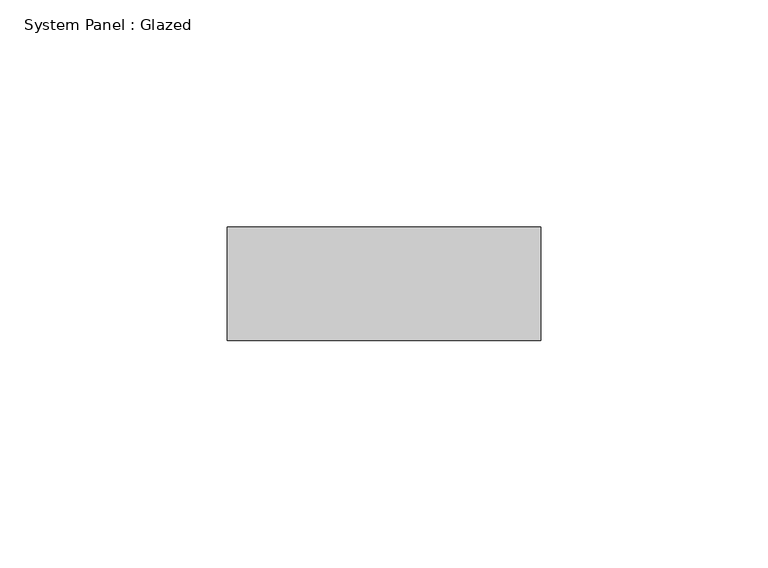
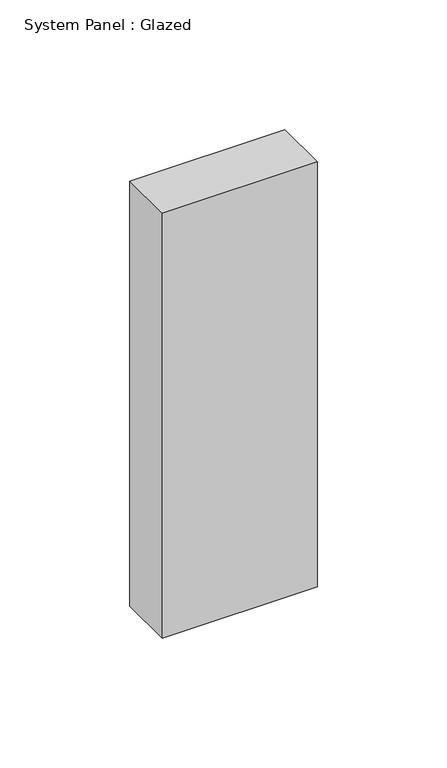
"""IFC4 building model written with IfcOpenShell, lengths in millimetres: plate geometry, System Panel : Glazed."""

import ifcopenshell
import ifcopenshell.guid

model = None  # the IFC model being written
_history = None  # IfcOwnerHistory: only IFC2X3 demands one
_inside = {}  # id of a spatial element -> (the spatial element, [elements in it])
_under = {}  # id of a project, library or spatial element -> (it, [spatial elements below it])
_declared = {}  # id of a project -> (the project, [libraries it declares])
_typed = {}  # id of a type object -> (the type object, [elements of that type])
_made_of = {}  # id of a material, layer set ... -> (it, [elements and type objects made of it])


def new_model(schema):
    """Start an empty IFC model of exactly this schema.

    Asked for "IFC4X3", IfcOpenShell would pick the latest addendum, in which some entities
    have other attributes; the version numbers below select the first issue.
    IFC2X3 requires an IfcOwnerHistory on every rooted entity: one is made here for all.
    """
    global model, _history
    if schema == "IFC4X3":
        model = ifcopenshell.file(schema_version=(4, 3, 0, 0))
    else:
        model = ifcopenshell.file(schema=schema)
    _inside.clear()
    _under.clear()
    _declared.clear()
    _typed.clear()
    _made_of.clear()
    _history = None
    if model.schema == "IFC2X3":
        org = make("IfcOrganization", Name="unknown")
        user = make(
            "IfcPersonAndOrganization",
            ThePerson=make("IfcPerson", FamilyName="unknown"),
            TheOrganization=org,
        )
        app = make(
            "IfcApplication",
            ApplicationDeveloper=org,
            Version="unknown",
            ApplicationFullName="unknown",
            ApplicationIdentifier="unknown",
        )
        _history = make(
            "IfcOwnerHistory",
            OwningUser=user,
            OwningApplication=app,
            ChangeAction="ADDED",
            CreationDate=0,
        )
    return model


def make(cls, **values):
    """One entity of the class cls with the attributes given. An attribute that is None is left unset."""
    return model.create_entity(
        cls, **{name: value for name, value in values.items() if value is not None}
    )


def rooted(cls, **values):
    """An entity with a GlobalId (a new one), such as an element, a storey or a relation."""
    return make(cls, GlobalId=ifcopenshell.guid.new(), OwnerHistory=_history, **values)


def si_unit(unit_type, name, prefix=None):
    """IfcSIUnit, for example si_unit("LENGTHUNIT", "METRE", prefix="MILLI")."""
    return make("IfcSIUnit", UnitType=unit_type, Prefix=prefix, Name=name)


def assignment(units):
    """IfcUnitAssignment: the units of a project."""
    return None if units is None else make("IfcUnitAssignment", Units=units)


def point(xyz):
    """IfcCartesianPoint."""
    return None if xyz is None else make("IfcCartesianPoint", Coordinates=xyz)


def direction(xyz):
    """IfcDirection."""
    return None if xyz is None else make("IfcDirection", DirectionRatios=xyz)


def frame(location, z_axis=None, x_axis=None):
    """IfcAxis2Placement3D, a coordinate frame: its origin and axes. An axis left out is left unset."""
    return make(
        "IfcAxis2Placement3D",
        Location=point(location),
        Axis=direction(z_axis),
        RefDirection=direction(x_axis),
    )


def origin():
    """The frame at (0, 0, 0) with its axes left unset."""
    return frame((0.0, 0.0, 0.0))


def origin_with_axes():
    """The frame at (0, 0, 0) with the z axis (0, 0, 1) and the x axis (1, 0, 0) written out."""
    return frame((0.0, 0.0, 0.0), z_axis=(0.0, 0.0, 1.0), x_axis=(1.0, 0.0, 0.0))


def place(relative_to, where):
    """IfcLocalPlacement: puts the frame where relative to a parent placement (None: the world)."""
    return make(
        "IfcLocalPlacement", PlacementRelTo=relative_to, RelativePlacement=where
    )


def context(
    kind, dimensions, precision=None, world=None, true_north=None, identifier=None
):
    """IfcGeometricRepresentationContext, for example the 3D "Model" context."""
    return make(
        "IfcGeometricRepresentationContext",
        ContextIdentifier=identifier,
        ContextType=kind,
        CoordinateSpaceDimension=dimensions,
        Precision=precision,
        WorldCoordinateSystem=world,
        TrueNorth=true_north,
    )


def project(units=None, contexts=None):
    """IfcProject with its units and contexts."""
    return rooted(
        "IfcProject",
        Name="project",
        RepresentationContexts=contexts,
        UnitsInContext=assignment(units),
    )


def spatial(cls, under=None, at=None, **own):
    """A site, building, storey or space (cls), placed at a placement, below another one or the project."""
    s = rooted(cls, ObjectPlacement=at, **own)
    if under is not None:
        _under.setdefault(under.id(), (under, []))[1].append(s)
    return s


def polyline(points):
    """IfcPolyline through the points."""
    return make("IfcPolyline", Points=[point(p) for p in points])


def outline(outer, holes=None, kind="AREA"):
    """IfcArbitraryClosedProfileDef: a profile drawn as a closed curve; with holes, ...WithVoids."""
    if holes is None:
        return make("IfcArbitraryClosedProfileDef", ProfileType=kind, OuterCurve=outer)
    return make(
        "IfcArbitraryProfileDefWithVoids",
        ProfileType=kind,
        OuterCurve=outer,
        InnerCurves=holes,
    )


def extrude(swept, where, along, depth):
    """IfcExtrudedAreaSolid: the profile swept, set in the frame where, extruded along a direction by depth."""
    return make(
        "IfcExtrudedAreaSolid",
        SweptArea=swept,
        Position=where,
        ExtrudedDirection=direction(along),
        Depth=depth,
    )


def shape(context_of_items, identifier, shape_type, items):
    """IfcShapeRepresentation: the items that make up one representation, for example the "Body"."""
    return make(
        "IfcShapeRepresentation",
        ContextOfItems=context_of_items,
        RepresentationIdentifier=identifier,
        RepresentationType=shape_type,
        Items=items,
    )


def source(mapping_origin, context_of_items, identifier, shape_type, items):
    """IfcRepresentationMap: a shape defined once, which mapped items show again and again."""
    return make(
        "IfcRepresentationMap",
        MappingOrigin=mapping_origin,
        MappedRepresentation=shape(context_of_items, identifier, shape_type, items),
    )


def transform(
    local_origin,
    x_axis=None,
    y_axis=None,
    z_axis=None,
    scale=None,
    scale2=None,
    scale3=None,
    uniform=True,
):
    """IfcCartesianTransformationOperator3D, or its non-uniform kind. x_axis, y_axis, z_axis: its Axis1, 2, 3."""
    if uniform:
        return make(
            "IfcCartesianTransformationOperator3D",
            Axis1=direction(x_axis),
            Axis2=direction(y_axis),
            LocalOrigin=point(local_origin),
            Scale=scale,
            Axis3=direction(z_axis),
        )
    return make(
        "IfcCartesianTransformationOperator3DnonUniform",
        Axis1=direction(x_axis),
        Axis2=direction(y_axis),
        LocalOrigin=point(local_origin),
        Scale=scale,
        Axis3=direction(z_axis),
        Scale2=scale2,
        Scale3=scale3,
    )


def mapped(mapping_source, mapping_target):
    """IfcMappedItem: shows the shape of a source again, moved by a transform."""
    return make(
        "IfcMappedItem", MappingSource=mapping_source, MappingTarget=mapping_target
    )


def made_of(thing, what):
    """Note that an element or type object is made of a material, layer set ...; save() writes the relation."""
    if what is not None:
        _made_of.setdefault(what.id(), (what, []))[1].append(thing)
    return thing


def element(
    cls,
    number,
    at=None,
    inside=None,
    cuts=None,
    type_object=None,
    material=None,
    context=None,
    identifier="Body",
    shape_type=None,
    held_by="IfcProductDefinitionShape",
    body=None,
    shapes=None,
    **own,
):
    """One element of the class cls, such as IfcWall. Its Tag is "e" and its number.

    at: its placement. inside: the storey or other place that contains it. cuts: it is an
    opening in that element (IfcRelVoidsElement). A single representation is given by context,
    identifier, shape_type and body (its items); several are given by shapes. held_by: the class
    of the entity that holds the representations. save() writes the other relations.
    """
    e = rooted(cls, Tag="e%d" % number, ObjectPlacement=at, **own)
    if body is not None:
        shapes = [shape(context, identifier, shape_type, body)]
    if shapes is not None:
        e.Representation = make(held_by, Representations=shapes)
    if inside is not None:
        _inside.setdefault(inside.id(), (inside, []))[1].append(e)
    if cuts is not None:
        rooted(
            "IfcRelVoidsElement", RelatingBuildingElement=cuts, RelatedOpeningElement=e
        )
    if type_object is not None:
        _typed.setdefault(type_object.id(), (type_object, []))[1].append(e)
    return made_of(e, material)


def aggregate(whole, parts):
    """IfcRelAggregates: a whole, such as a stair, and the parts it consists of."""
    return rooted("IfcRelAggregates", RelatingObject=whole, RelatedObjects=parts)


def save(model, path):
    """Write the relations noted so far, then the file.

    IfcRelAggregates (storeys below a building ...), IfcRelContainedInSpatialStructure (elements
    in a storey), IfcRelDefinesByType, IfcRelAssociatesMaterial and IfcRelDeclares: one each for
    every whole, place, type object, material and project.
    """
    for whole, parts in _under.values():
        aggregate(whole, parts)
    for where, things in _inside.values():
        rooted(
            "IfcRelContainedInSpatialStructure",
            RelatedElements=things,
            RelatingStructure=where,
        )
    for kind, things in _typed.values():
        rooted("IfcRelDefinesByType", RelatedObjects=things, RelatingType=kind)
    for what, things in _made_of.values():
        rooted("IfcRelAssociatesMaterial", RelatedObjects=things, RelatingMaterial=what)
    for by, libraries in _declared.values():
        rooted("IfcRelDeclares", RelatingContext=by, RelatedDefinitions=libraries)
    model.write(path)


def system_panel_glazed_efe9a4c3(model_context):
    return source(origin(), model_context, "Body", "SweptSolid", [
        extrude(outline(polyline([(34.4971749, 24.5), (-34.4971749, 24.5), (-34.4971749, 49.5), (34.4971749, 49.5), (34.4971749, 24.5)])), origin_with_axes(), (0.0, 0.0, 1.0), 200.0),
    ])


if __name__ == "__main__":
    model = new_model("IFC4")
    model_context = context("Model", 3, world=origin())
    ifc_project = project(units=[si_unit("LENGTHUNIT", "METRE", prefix="MILLI")], contexts=[model_context])
    site = spatial("IfcSite", under=ifc_project)
    building = spatial("IfcBuilding", under=site)
    placement = place(None, origin())
    system_panel_glazed_shape = system_panel_glazed_efe9a4c3(model_context)
    element("IfcPlate", 1, ObjectType="System Panel : Glazed", at=placement, inside=building, context=model_context, shape_type="MappedRepresentation", body=[
        mapped(system_panel_glazed_shape, transform((0.0, 0.0, 0.0), x_axis=(1.0, 0.0, 0.0), y_axis=(0.0, 1.0, 0.0), z_axis=(0.0, 0.0, 1.0))),
    ])
    save(model, "model.ifc")

# Revit data of these elements
# Element 1 (IfcPlate, "System Panel : Glazed")
#   Materials on its faces: "Glass"
# Materials
#   "Glass": class "Glass", colour RGB 218 227 224, transparency 0.85, Description = "Soda Lime Glass", Cost = 0
